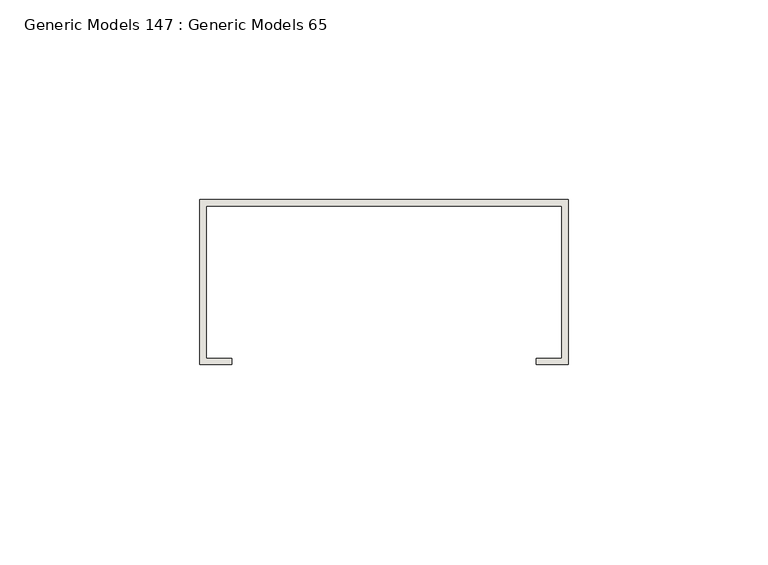
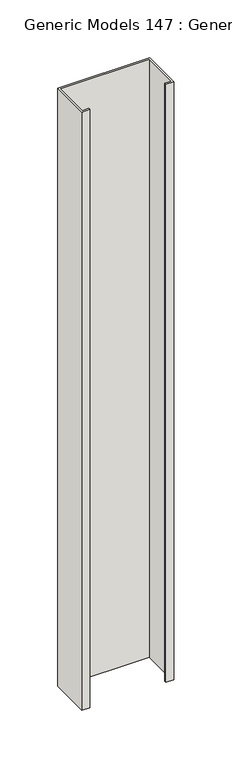
"""IFC4 building model written with IfcOpenShell, lengths in millimetres: wall geometry, Generic Models 147 : Generic Models 65."""

from ifc_helpers import new_model, si_unit, frame, origin, place, context, project, spatial, polyline, outline, extrude, source, transform, mapped, element, save


def generic_models_147_generic_models_65_0860e088(model_context):
    return source(origin(), model_context, "Body", "SweptSolid", [
        extrude(outline(polyline([(50911.125, 630.2375), (51003.2, 630.2375), (51003.2, 588.9625), (50995.2625, 588.9625), (50995.2625, 590.55), (51001.6125, 590.55), (51001.6125, 628.65), (50912.7125, 628.65), (50912.7125, 590.55), (50919.0625, 590.55), (50919.0625, 588.9625), (50911.125, 588.9625), (50911.125, 630.2375)])), frame((0.0, 0.0, 1824.2359375), z_axis=(0.0, 0.0, 1.0), x_axis=(1.0, 0.0, 0.0)), (0.0, 0.0, 1.0), 631.6265625),
    ])


if __name__ == "__main__":
    model = new_model("IFC4")
    model_context = context("Model", 3, world=origin())
    ifc_project = project(units=[si_unit("LENGTHUNIT", "METRE", prefix="MILLI")], contexts=[model_context])
    site = spatial("IfcSite", under=ifc_project)
    building = spatial("IfcBuilding", under=site)
    placement = place(None, origin())
    generic_models_147_generic_models_65_shape = generic_models_147_generic_models_65_0860e088(model_context)
    element("IfcWall", 1, ObjectType="Generic Models 147 : Generic Models 65", at=placement, inside=building, context=model_context, shape_type="MappedRepresentation", body=[
        mapped(generic_models_147_generic_models_65_shape, transform((0.0, 0.0, 0.0), x_axis=(1.0, 0.0, 0.0), y_axis=(0.0, 1.0, 0.0), z_axis=(0.0, 0.0, 1.0))),
    ])
    save(model, "model.ifc")

# Revit data of these elements
# Element 1 (IfcWall, "Generic Models 147 : Generic Models 65")
#   Materials on its faces: "METAL STUD (16\" O.C.)"
# Materials
#   "METAL STUD (16\" O.C.)": class "Unassigned", colour RGB 210 209 208, transparency 0, Keynote = "M05121300.02", Cost = 0
